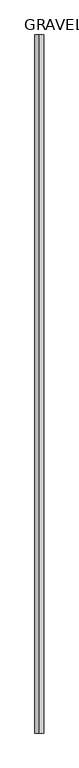
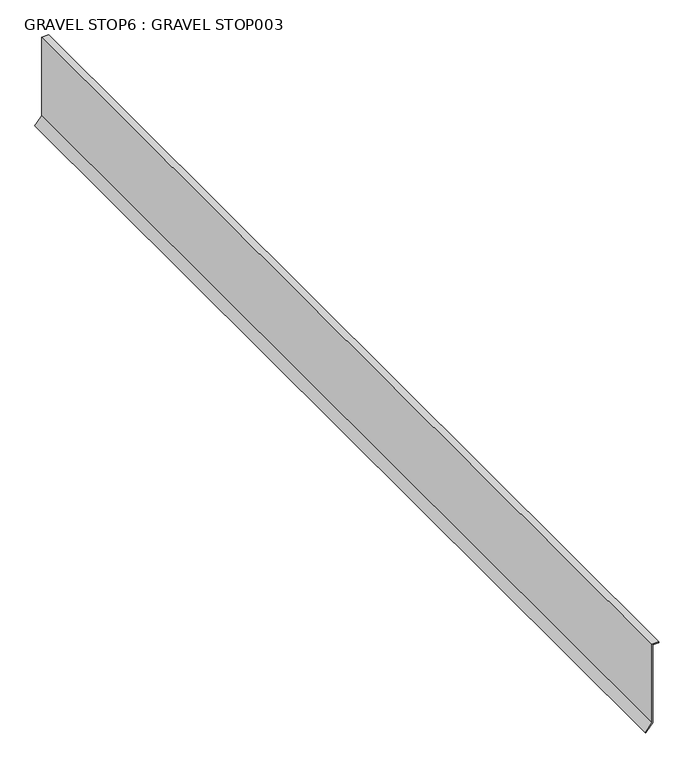
"""IFC4 building model written with IfcOpenShell, lengths in millimetres: proxy geometry, GRAVEL STOP6 : GRAVEL STOP003."""

from ifc_helpers import new_model, si_unit, frame, origin, place, context, project, spatial, polyline, outline, extrude, source, transform, mapped, element, save


def gravel_stop6_gravel_stop003_73d50619(model_context):
    return source(origin(), model_context, "Body", "SweptSolid", [
        extrude(outline(polyline([(40082.2407116, -5046.164524), (40081.3605882, -5045.0615204), (40097.4918556, -5032.189842), (40253.3245993, -5032.189842), (40253.3245993, -5020.4219233), (40254.7357103, -5020.4219233), (40254.7357103, -5033.600953), (40097.9858473, -5033.600953), (40082.2407116, -5046.164524)])), frame((0.0, -1052.8906573, 0.0), z_axis=(0.0, 1.0, 0.0), x_axis=(0.0, 0.0, 1.0)), (0.0, 0.0, 1.0), 2000.25),
    ])


if __name__ == "__main__":
    model = new_model("IFC4")
    model_context = context("Model", 3, world=origin())
    ifc_project = project(units=[si_unit("LENGTHUNIT", "METRE", prefix="MILLI")], contexts=[model_context])
    site = spatial("IfcSite", under=ifc_project)
    building = spatial("IfcBuilding", under=site)
    placement = place(None, origin())
    gravel_stop6_gravel_stop003_shape = gravel_stop6_gravel_stop003_73d50619(model_context)
    element("IfcBuildingElementProxy", 1, Name="GRAVEL STOP6 : GRAVEL STOP003", ObjectType="GRAVEL STOP6 : GRAVEL STOP003", at=placement, inside=building, context=model_context, shape_type="MappedRepresentation", body=[
        mapped(gravel_stop6_gravel_stop003_shape, transform((0.0, 0.0, 0.0), x_axis=(1.0, 0.0, 0.0), y_axis=(0.0, 1.0, 0.0), z_axis=(0.0, 0.0, 1.0))),
    ])
    save(model, "model.ifc")

# Revit data of these elements
# Type "GRAVEL STOP6 : GRAVEL STOP003"
#   NameOverride = "GRAVEL STOP003"
# Element 1 (IfcBuildingElementProxy, "GRAVEL STOP6 : GRAVEL STOP003")
#   Materials on its faces: "GRAVEL STOP REQUIRED WITH GRAVEL SURFACE SYSTEMS"
# Materials
#   "GRAVEL STOP REQUIRED WITH GRAVEL SURFACE SYSTEMS": class "Unassigned", colour RGB 170 170 127, transparency 0, Cost = 0
